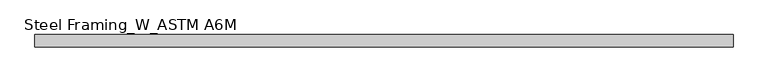
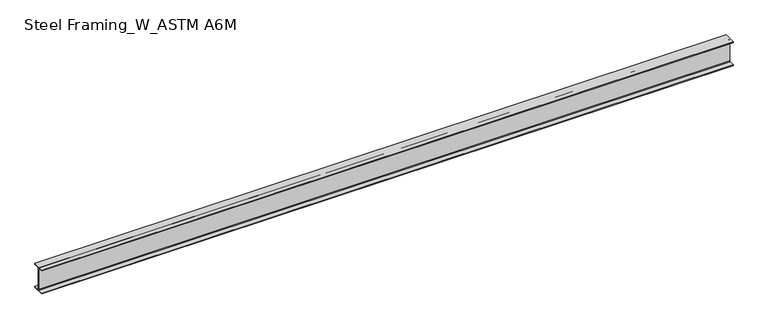
"""IFC4 building model written with IfcOpenShell, lengths in millimetres: beam geometry, Steel Framing_W_ASTM A6M : H_SB_AR_S02_W360x51_B4."""

import ifcopenshell
import ifcopenshell.guid

model = None  # the IFC model being written
_history = None  # IfcOwnerHistory: only IFC2X3 demands one
_inside = {}  # id of a spatial element -> (the spatial element, [elements in it])
_under = {}  # id of a project, library or spatial element -> (it, [spatial elements below it])
_declared = {}  # id of a project -> (the project, [libraries it declares])
_typed = {}  # id of a type object -> (the type object, [elements of that type])
_made_of = {}  # id of a material, layer set ... -> (it, [elements and type objects made of it])


def new_model(schema):
    """Start an empty IFC model of exactly this schema.

    Asked for "IFC4X3", IfcOpenShell would pick the latest addendum, in which some entities
    have other attributes; the version numbers below select the first issue.
    IFC2X3 requires an IfcOwnerHistory on every rooted entity: one is made here for all.
    """
    global model, _history
    if schema == "IFC4X3":
        model = ifcopenshell.file(schema_version=(4, 3, 0, 0))
    else:
        model = ifcopenshell.file(schema=schema)
    _inside.clear()
    _under.clear()
    _declared.clear()
    _typed.clear()
    _made_of.clear()
    _history = None
    if model.schema == "IFC2X3":
        org = make("IfcOrganization", Name="unknown")
        user = make(
            "IfcPersonAndOrganization",
            ThePerson=make("IfcPerson", FamilyName="unknown"),
            TheOrganization=org,
        )
        app = make(
            "IfcApplication",
            ApplicationDeveloper=org,
            Version="unknown",
            ApplicationFullName="unknown",
            ApplicationIdentifier="unknown",
        )
        _history = make(
            "IfcOwnerHistory",
            OwningUser=user,
            OwningApplication=app,
            ChangeAction="ADDED",
            CreationDate=0,
        )
    return model


def make(cls, **values):
    """One entity of the class cls with the attributes given. An attribute that is None is left unset."""
    return model.create_entity(
        cls, **{name: value for name, value in values.items() if value is not None}
    )


def rooted(cls, **values):
    """An entity with a GlobalId (a new one), such as an element, a storey or a relation."""
    return make(cls, GlobalId=ifcopenshell.guid.new(), OwnerHistory=_history, **values)


def si_unit(unit_type, name, prefix=None):
    """IfcSIUnit, for example si_unit("LENGTHUNIT", "METRE", prefix="MILLI")."""
    return make("IfcSIUnit", UnitType=unit_type, Prefix=prefix, Name=name)


def assignment(units):
    """IfcUnitAssignment: the units of a project."""
    return None if units is None else make("IfcUnitAssignment", Units=units)


def point(xyz):
    """IfcCartesianPoint."""
    return None if xyz is None else make("IfcCartesianPoint", Coordinates=xyz)


def direction(xyz):
    """IfcDirection."""
    return None if xyz is None else make("IfcDirection", DirectionRatios=xyz)


def frame(location, z_axis=None, x_axis=None):
    """IfcAxis2Placement3D, a coordinate frame: its origin and axes. An axis left out is left unset."""
    return make(
        "IfcAxis2Placement3D",
        Location=point(location),
        Axis=direction(z_axis),
        RefDirection=direction(x_axis),
    )


def frame_2d(location, x_axis=None):
    """IfcAxis2Placement2D, a coordinate frame in the plane: its origin and x axis."""
    return make(
        "IfcAxis2Placement2D", Location=point(location), RefDirection=direction(x_axis)
    )


def origin():
    """The frame at (0, 0, 0) with its axes left unset."""
    return frame((0.0, 0.0, 0.0))


def place(relative_to, where):
    """IfcLocalPlacement: puts the frame where relative to a parent placement (None: the world)."""
    return make(
        "IfcLocalPlacement", PlacementRelTo=relative_to, RelativePlacement=where
    )


def context(
    kind, dimensions, precision=None, world=None, true_north=None, identifier=None
):
    """IfcGeometricRepresentationContext, for example the 3D "Model" context."""
    return make(
        "IfcGeometricRepresentationContext",
        ContextIdentifier=identifier,
        ContextType=kind,
        CoordinateSpaceDimension=dimensions,
        Precision=precision,
        WorldCoordinateSystem=world,
        TrueNorth=true_north,
    )


def project(units=None, contexts=None):
    """IfcProject with its units and contexts."""
    return rooted(
        "IfcProject",
        Name="project",
        RepresentationContexts=contexts,
        UnitsInContext=assignment(units),
    )


def spatial(cls, under=None, at=None, **own):
    """A site, building, storey or space (cls), placed at a placement, below another one or the project."""
    s = rooted(cls, ObjectPlacement=at, **own)
    if under is not None:
        _under.setdefault(under.id(), (under, []))[1].append(s)
    return s


def polyline(points):
    """IfcPolyline through the points."""
    return make("IfcPolyline", Points=[point(p) for p in points])


def circle_curve(where, radius):
    """IfcCircle in the frame where."""
    return make("IfcCircle", Position=where, Radius=radius)


def trimmed(basis, trim1, trim2, sense, master):
    """IfcTrimmedCurve: the piece of a basis curve between two trims."""
    return make(
        "IfcTrimmedCurve",
        BasisCurve=basis,
        Trim1=trim1,
        Trim2=trim2,
        SenseAgreement=sense,
        MasterRepresentation=master,
    )


def segment(curve, same_sense, transition):
    """IfcCompositeCurveSegment."""
    return make(
        "IfcCompositeCurveSegment",
        Transition=transition,
        SameSense=same_sense,
        ParentCurve=curve,
    )


def composite_curve(segments, self_intersect=None):
    """IfcCompositeCurve: segments joined end to end."""
    return make("IfcCompositeCurve", Segments=segments, SelfIntersect=self_intersect)


def outline(outer, holes=None, kind="AREA"):
    """IfcArbitraryClosedProfileDef: a profile drawn as a closed curve; with holes, ...WithVoids."""
    if holes is None:
        return make("IfcArbitraryClosedProfileDef", ProfileType=kind, OuterCurve=outer)
    return make(
        "IfcArbitraryProfileDefWithVoids",
        ProfileType=kind,
        OuterCurve=outer,
        InnerCurves=holes,
    )


def extrude(swept, where, along, depth):
    """IfcExtrudedAreaSolid: the profile swept, set in the frame where, extruded along a direction by depth."""
    return make(
        "IfcExtrudedAreaSolid",
        SweptArea=swept,
        Position=where,
        ExtrudedDirection=direction(along),
        Depth=depth,
    )


def shape(context_of_items, identifier, shape_type, items):
    """IfcShapeRepresentation: the items that make up one representation, for example the "Body"."""
    return make(
        "IfcShapeRepresentation",
        ContextOfItems=context_of_items,
        RepresentationIdentifier=identifier,
        RepresentationType=shape_type,
        Items=items,
    )


def source(mapping_origin, context_of_items, identifier, shape_type, items):
    """IfcRepresentationMap: a shape defined once, which mapped items show again and again."""
    return make(
        "IfcRepresentationMap",
        MappingOrigin=mapping_origin,
        MappedRepresentation=shape(context_of_items, identifier, shape_type, items),
    )


def transform(
    local_origin,
    x_axis=None,
    y_axis=None,
    z_axis=None,
    scale=None,
    scale2=None,
    scale3=None,
    uniform=True,
):
    """IfcCartesianTransformationOperator3D, or its non-uniform kind. x_axis, y_axis, z_axis: its Axis1, 2, 3."""
    if uniform:
        return make(
            "IfcCartesianTransformationOperator3D",
            Axis1=direction(x_axis),
            Axis2=direction(y_axis),
            LocalOrigin=point(local_origin),
            Scale=scale,
            Axis3=direction(z_axis),
        )
    return make(
        "IfcCartesianTransformationOperator3DnonUniform",
        Axis1=direction(x_axis),
        Axis2=direction(y_axis),
        LocalOrigin=point(local_origin),
        Scale=scale,
        Axis3=direction(z_axis),
        Scale2=scale2,
        Scale3=scale3,
    )


def mapped(mapping_source, mapping_target):
    """IfcMappedItem: shows the shape of a source again, moved by a transform."""
    return make(
        "IfcMappedItem", MappingSource=mapping_source, MappingTarget=mapping_target
    )


def made_of(thing, what):
    """Note that an element or type object is made of a material, layer set ...; save() writes the relation."""
    if what is not None:
        _made_of.setdefault(what.id(), (what, []))[1].append(thing)
    return thing


def element(
    cls,
    number,
    at=None,
    inside=None,
    cuts=None,
    type_object=None,
    material=None,
    context=None,
    identifier="Body",
    shape_type=None,
    held_by="IfcProductDefinitionShape",
    body=None,
    shapes=None,
    **own,
):
    """One element of the class cls, such as IfcWall. Its Tag is "e" and its number.

    at: its placement. inside: the storey or other place that contains it. cuts: it is an
    opening in that element (IfcRelVoidsElement). A single representation is given by context,
    identifier, shape_type and body (its items); several are given by shapes. held_by: the class
    of the entity that holds the representations. save() writes the other relations.
    """
    e = rooted(cls, Tag="e%d" % number, ObjectPlacement=at, **own)
    if body is not None:
        shapes = [shape(context, identifier, shape_type, body)]
    if shapes is not None:
        e.Representation = make(held_by, Representations=shapes)
    if inside is not None:
        _inside.setdefault(inside.id(), (inside, []))[1].append(e)
    if cuts is not None:
        rooted(
            "IfcRelVoidsElement", RelatingBuildingElement=cuts, RelatedOpeningElement=e
        )
    if type_object is not None:
        _typed.setdefault(type_object.id(), (type_object, []))[1].append(e)
    return made_of(e, material)


def aggregate(whole, parts):
    """IfcRelAggregates: a whole, such as a stair, and the parts it consists of."""
    return rooted("IfcRelAggregates", RelatingObject=whole, RelatedObjects=parts)


def save(model, path):
    """Write the relations noted so far, then the file.

    IfcRelAggregates (storeys below a building ...), IfcRelContainedInSpatialStructure (elements
    in a storey), IfcRelDefinesByType, IfcRelAssociatesMaterial and IfcRelDeclares: one each for
    every whole, place, type object, material and project.
    """
    for whole, parts in _under.values():
        aggregate(whole, parts)
    for where, things in _inside.values():
        rooted(
            "IfcRelContainedInSpatialStructure",
            RelatedElements=things,
            RelatingStructure=where,
        )
    for kind, things in _typed.values():
        rooted("IfcRelDefinesByType", RelatedObjects=things, RelatingType=kind)
    for what, things in _made_of.values():
        rooted("IfcRelAssociatesMaterial", RelatedObjects=things, RelatingMaterial=what)
    for by, libraries in _declared.values():
        rooted("IfcRelDeclares", RelatingContext=by, RelatedDefinitions=libraries)
    model.write(path)


def steel_framing_w_astm_a6m_8e55c2dc(model_context):
    return source(origin(), model_context, "Body", "SweptSolid", [
        extrude(outline(composite_curve([segment(polyline([(85.5, -166.4), (85.5, -178.0), (-85.5, -178.0), (-85.5, -166.4), (-13.72, -166.4)]), True, "CONTINUOUS"), segment(trimmed(circle_curve(frame_2d((-13.72, -156.3)), 10.1), [point((-13.72, -166.4))], [point((-3.62, -156.3))], True, "CARTESIAN"), True, "CONTINUOUS"), segment(polyline([(-3.62, -156.3), (-3.62, 156.3)]), True, "CONTINUOUS"), segment(trimmed(circle_curve(frame_2d((-13.72, 156.3)), 10.1), [point((-3.62, 156.3))], [point((-13.72, 166.4))], True, "CARTESIAN"), True, "CONTINUOUS"), segment(polyline([(-13.72, 166.4), (-85.5, 166.4), (-85.5, 178.0), (85.5, 178.0), (85.5, 166.4), (13.72, 166.4)]), True, "CONTINUOUS"), segment(trimmed(circle_curve(frame_2d((13.72, 156.3)), 10.1), [point((13.72, 166.4))], [point((3.62, 156.3))], True, "CARTESIAN"), True, "CONTINUOUS"), segment(polyline([(3.62, 156.3), (3.62, -156.3)]), True, "CONTINUOUS"), segment(trimmed(circle_curve(frame_2d((13.72, -156.3)), 10.1), [point((3.62, -156.3))], [point((13.72, -166.4))], True, "CARTESIAN"), True, "CONTINUOUS"), segment(polyline([(13.72, -166.4), (85.5, -166.4)]), True, "CONTINUOUS")], self_intersect=False)), frame((-4901.8, 0.0, 0.0), z_axis=(1.0, 0.0, 0.0), x_axis=(0.0, 1.0, 0.0)), (0.0, 0.0, 1.0), 9803.6),
    ])


if __name__ == "__main__":
    model = new_model("IFC4")
    model_context = context("Model", 3, world=origin())
    ifc_project = project(units=[si_unit("LENGTHUNIT", "METRE", prefix="MILLI")], contexts=[model_context])
    site = spatial("IfcSite", under=ifc_project)
    building = spatial("IfcBuilding", under=site)
    placement = place(None, origin())
    steel_framing_w_astm_a6m_shape = steel_framing_w_astm_a6m_8e55c2dc(model_context)
    element("IfcBeam", 1, ObjectType="Steel Framing_W_ASTM A6M : H_SB_AR_S02_W360x51_B4", at=placement, inside=building, context=model_context, shape_type="MappedRepresentation", body=[
        mapped(steel_framing_w_astm_a6m_shape, transform((0.0, 0.0, 0.0), x_axis=(1.0, 0.0, 0.0), y_axis=(0.0, 1.0, 0.0), z_axis=(0.0, 0.0, 1.0))),
    ])
    save(model, "model.ifc")

# Revit data of these elements
# Type "Steel Framing_W_ASTM A6M : H_SB_AR_S02_W360x51_B4"
#   Type Mark = "B4"
#   Section Name Key = "W14x34"
#   Width = 17.1 cm
#   Web Thickness = 0.724 cm
#   Web Fillet = 1.01 cm
#   Warping Constant = 287000.0 cm⁶
#   Torsional Moment of Inertia = 23.70 cm⁴
#   Section Area = 64.5 cm²
#   Plastic Modulus weak axis = 174.0 cm³
#   Plastic Modulus strong axis = 895.0 cm³
#   Perimeter = 1.36 m²/m
#   Nominal Weight = 51.00 kgf/m
#   Moment of Inertia weak axis = 970.00 cm⁴
#   Moment of Inertia strong axis = 14200.00 cm⁴
#   Height = 35.6 cm
#   Flange Thickness = 1.16 cm
#   Elastic Modulus weak axis = 113.0 cm³
#   Elastic Modulus strong axis = 796.0 cm³
#   Centroid Vertical = 17.8 cm
#   Centroid Horizontal = 8.55 cm
#   Length [instance default] = 1500 mm
#   Structural Material [instance default] = Steel, 45-345
#   Bolt Spacing = 0
#   Assembly Code = ""
# Element 1 (IfcBeam, "Steel Framing_W_ASTM A6M : H_SB_AR_S02_W360x51_B4")
#   Materials on its faces: "Steel, 45-345"
# Materials
#   "Steel, 45-345": class "Metal", colour RGB 189 187 185, transparency 0, Description = "Steel 345 MPa", Cost = 0
